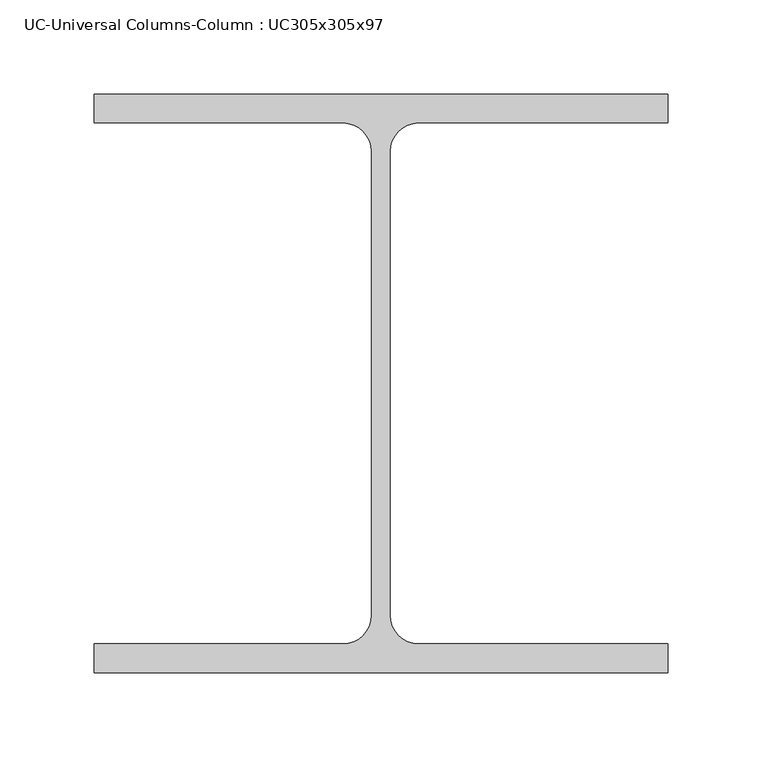
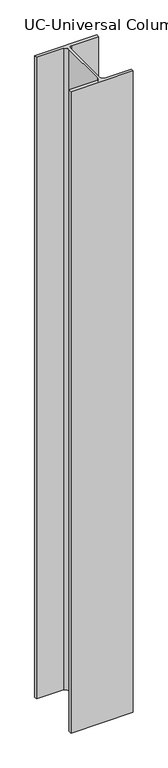
"""IFC4 building model written with IfcOpenShell, lengths in millimetres: column geometry, UC-Universal Columns-Column : UC305x305x97."""

from ifc_helpers import new_model, si_unit, point, frame_2d, origin, origin_with_axes, place, context, project, spatial, polyline, circle_curve, trimmed, segment, composite_curve, outline, extrude, source, transform, mapped, element, save


def uc_universal_columns_column_uc305x305x97_559dd73d(model_context):
    return source(origin(), model_context, "Body", "SweptSolid", [
        extrude(outline(composite_curve([segment(polyline([(152.65, 153.95), (152.65, 138.55), (20.15, 138.55)]), True, "CONTINUOUS"), segment(trimmed(circle_curve(frame_2d((20.15, 123.35)), 15.2), [point((20.15, 138.55))], [point((4.95, 123.35))], True, "CARTESIAN"), True, "CONTINUOUS"), segment(polyline([(4.95, 123.35), (4.95, -123.35)]), True, "CONTINUOUS"), segment(trimmed(circle_curve(frame_2d((20.15, -123.35)), 15.2), [point((4.95, -123.35))], [point((20.15, -138.55))], True, "CARTESIAN"), True, "CONTINUOUS"), segment(polyline([(20.15, -138.55), (152.65, -138.55), (152.65, -153.95), (-152.65, -153.95), (-152.65, -138.55), (-20.15, -138.55)]), True, "CONTINUOUS"), segment(trimmed(circle_curve(frame_2d((-20.15, -123.35)), 15.2), [point((-20.15, -138.55))], [point((-4.95, -123.35))], True, "CARTESIAN"), True, "CONTINUOUS"), segment(polyline([(-4.95, -123.35), (-4.95, 123.35)]), True, "CONTINUOUS"), segment(trimmed(circle_curve(frame_2d((-20.15, 123.35)), 15.2), [point((-4.95, 123.35))], [point((-20.15, 138.55))], True, "CARTESIAN"), True, "CONTINUOUS"), segment(polyline([(-20.15, 138.55), (-152.65, 138.55), (-152.65, 153.95), (152.65, 153.95)]), True, "CONTINUOUS")], self_intersect=False)), origin_with_axes(), (0.0, 0.0, 1.0), 3327.4),
    ])


if __name__ == "__main__":
    model = new_model("IFC4")
    model_context = context("Model", 3, world=origin())
    ifc_project = project(units=[si_unit("LENGTHUNIT", "METRE", prefix="MILLI")], contexts=[model_context])
    site = spatial("IfcSite", under=ifc_project)
    building = spatial("IfcBuilding", under=site)
    placement = place(None, origin())
    uc_universal_columns_column_uc305x305x97_shape = uc_universal_columns_column_uc305x305x97_559dd73d(model_context)
    element("IfcColumn", 1, ObjectType="UC-Universal Columns-Column : UC305x305x97", at=placement, inside=building, context=model_context, shape_type="MappedRepresentation", body=[
        mapped(uc_universal_columns_column_uc305x305x97_shape, transform((0.0, 0.0, 0.0), x_axis=(1.0, 0.0, 0.0), y_axis=(0.0, 1.0, 0.0), z_axis=(0.0, 0.0, 1.0))),
    ])
    save(model, "model.ifc")

# Revit data of these elements
# Type "UC-Universal Columns-Column : UC305x305x97"
#   Section Name Key = "UC305x305x97"
#   Width = 30.53 cm
#   Web Thickness = 0.99 cm
#   Web Fillet = 1.52 cm
#   Warping Constant = 1560000.0 cm⁶
#   Torsional Moment of Inertia = 91.20 cm⁴
#   Section Area = 123.0 cm²
#   Plastic Modulus weak axis = 726.0 cm³
#   Plastic Modulus strong axis = 1592.0 cm³
#   Nominal Weight = 96.8996 kgf/m
#   Moment of Inertia weak axis = 7308.00 cm⁴
#   Moment of Inertia strong axis = 22249.00 cm⁴
#   Height = 30.79 cm
#   Flange Thickness = 1.54 cm
#   Elastic Modulus weak axis = 479.0 cm³
#   Elastic Modulus strong axis = 1445.0 cm³
#   Centroid Vertical = 15.395 cm
#   Centroid Horizontal = 15.265 cm
#   Bolt Spacing = 14.0 cm
#   Structural Material [instance default] = Metal - Steel 43-275
#   Type Comments = ""
#   Assembly Code = ""
# Element 1 (IfcColumn, "UC-Universal Columns-Column : UC305x305x97")
#   Materials on its faces: "Metal - Steel 43-275"
# Materials
#   "Metal - Steel 43-275": class "Metal", colour RGB 247 247 247, transparency 0, Cost = 0
